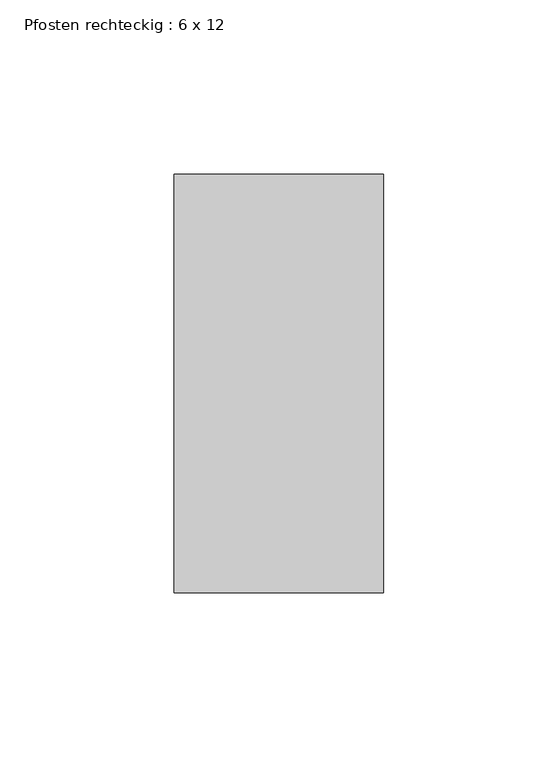
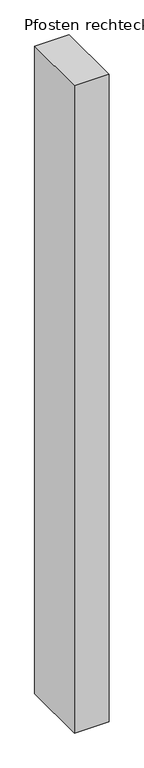
"""IFC4 building model written with IfcOpenShell, lengths in millimetres: member geometry, Pfosten rechteckig : 6 x 12."""

import ifcopenshell
import ifcopenshell.guid

model = None  # the IFC model being written
_history = None  # IfcOwnerHistory: only IFC2X3 demands one
_inside = {}  # id of a spatial element -> (the spatial element, [elements in it])
_under = {}  # id of a project, library or spatial element -> (it, [spatial elements below it])
_declared = {}  # id of a project -> (the project, [libraries it declares])
_typed = {}  # id of a type object -> (the type object, [elements of that type])
_made_of = {}  # id of a material, layer set ... -> (it, [elements and type objects made of it])


def new_model(schema):
    """Start an empty IFC model of exactly this schema.

    Asked for "IFC4X3", IfcOpenShell would pick the latest addendum, in which some entities
    have other attributes; the version numbers below select the first issue.
    IFC2X3 requires an IfcOwnerHistory on every rooted entity: one is made here for all.
    """
    global model, _history
    if schema == "IFC4X3":
        model = ifcopenshell.file(schema_version=(4, 3, 0, 0))
    else:
        model = ifcopenshell.file(schema=schema)
    _inside.clear()
    _under.clear()
    _declared.clear()
    _typed.clear()
    _made_of.clear()
    _history = None
    if model.schema == "IFC2X3":
        org = make("IfcOrganization", Name="unknown")
        user = make(
            "IfcPersonAndOrganization",
            ThePerson=make("IfcPerson", FamilyName="unknown"),
            TheOrganization=org,
        )
        app = make(
            "IfcApplication",
            ApplicationDeveloper=org,
            Version="unknown",
            ApplicationFullName="unknown",
            ApplicationIdentifier="unknown",
        )
        _history = make(
            "IfcOwnerHistory",
            OwningUser=user,
            OwningApplication=app,
            ChangeAction="ADDED",
            CreationDate=0,
        )
    return model


def make(cls, **values):
    """One entity of the class cls with the attributes given. An attribute that is None is left unset."""
    return model.create_entity(
        cls, **{name: value for name, value in values.items() if value is not None}
    )


def rooted(cls, **values):
    """An entity with a GlobalId (a new one), such as an element, a storey or a relation."""
    return make(cls, GlobalId=ifcopenshell.guid.new(), OwnerHistory=_history, **values)


def si_unit(unit_type, name, prefix=None):
    """IfcSIUnit, for example si_unit("LENGTHUNIT", "METRE", prefix="MILLI")."""
    return make("IfcSIUnit", UnitType=unit_type, Prefix=prefix, Name=name)


def assignment(units):
    """IfcUnitAssignment: the units of a project."""
    return None if units is None else make("IfcUnitAssignment", Units=units)


def point(xyz):
    """IfcCartesianPoint."""
    return None if xyz is None else make("IfcCartesianPoint", Coordinates=xyz)


def direction(xyz):
    """IfcDirection."""
    return None if xyz is None else make("IfcDirection", DirectionRatios=xyz)


def frame(location, z_axis=None, x_axis=None):
    """IfcAxis2Placement3D, a coordinate frame: its origin and axes. An axis left out is left unset."""
    return make(
        "IfcAxis2Placement3D",
        Location=point(location),
        Axis=direction(z_axis),
        RefDirection=direction(x_axis),
    )


def origin():
    """The frame at (0, 0, 0) with its axes left unset."""
    return frame((0.0, 0.0, 0.0))


def place(relative_to, where):
    """IfcLocalPlacement: puts the frame where relative to a parent placement (None: the world)."""
    return make(
        "IfcLocalPlacement", PlacementRelTo=relative_to, RelativePlacement=where
    )


def context(
    kind, dimensions, precision=None, world=None, true_north=None, identifier=None
):
    """IfcGeometricRepresentationContext, for example the 3D "Model" context."""
    return make(
        "IfcGeometricRepresentationContext",
        ContextIdentifier=identifier,
        ContextType=kind,
        CoordinateSpaceDimension=dimensions,
        Precision=precision,
        WorldCoordinateSystem=world,
        TrueNorth=true_north,
    )


def project(units=None, contexts=None):
    """IfcProject with its units and contexts."""
    return rooted(
        "IfcProject",
        Name="project",
        RepresentationContexts=contexts,
        UnitsInContext=assignment(units),
    )


def spatial(cls, under=None, at=None, **own):
    """A site, building, storey or space (cls), placed at a placement, below another one or the project."""
    s = rooted(cls, ObjectPlacement=at, **own)
    if under is not None:
        _under.setdefault(under.id(), (under, []))[1].append(s)
    return s


def polyline(points):
    """IfcPolyline through the points."""
    return make("IfcPolyline", Points=[point(p) for p in points])


def outline(outer, holes=None, kind="AREA"):
    """IfcArbitraryClosedProfileDef: a profile drawn as a closed curve; with holes, ...WithVoids."""
    if holes is None:
        return make("IfcArbitraryClosedProfileDef", ProfileType=kind, OuterCurve=outer)
    return make(
        "IfcArbitraryProfileDefWithVoids",
        ProfileType=kind,
        OuterCurve=outer,
        InnerCurves=holes,
    )


def extrude(swept, where, along, depth):
    """IfcExtrudedAreaSolid: the profile swept, set in the frame where, extruded along a direction by depth."""
    return make(
        "IfcExtrudedAreaSolid",
        SweptArea=swept,
        Position=where,
        ExtrudedDirection=direction(along),
        Depth=depth,
    )


def shape(context_of_items, identifier, shape_type, items):
    """IfcShapeRepresentation: the items that make up one representation, for example the "Body"."""
    return make(
        "IfcShapeRepresentation",
        ContextOfItems=context_of_items,
        RepresentationIdentifier=identifier,
        RepresentationType=shape_type,
        Items=items,
    )


def source(mapping_origin, context_of_items, identifier, shape_type, items):
    """IfcRepresentationMap: a shape defined once, which mapped items show again and again."""
    return make(
        "IfcRepresentationMap",
        MappingOrigin=mapping_origin,
        MappedRepresentation=shape(context_of_items, identifier, shape_type, items),
    )


def transform(
    local_origin,
    x_axis=None,
    y_axis=None,
    z_axis=None,
    scale=None,
    scale2=None,
    scale3=None,
    uniform=True,
):
    """IfcCartesianTransformationOperator3D, or its non-uniform kind. x_axis, y_axis, z_axis: its Axis1, 2, 3."""
    if uniform:
        return make(
            "IfcCartesianTransformationOperator3D",
            Axis1=direction(x_axis),
            Axis2=direction(y_axis),
            LocalOrigin=point(local_origin),
            Scale=scale,
            Axis3=direction(z_axis),
        )
    return make(
        "IfcCartesianTransformationOperator3DnonUniform",
        Axis1=direction(x_axis),
        Axis2=direction(y_axis),
        LocalOrigin=point(local_origin),
        Scale=scale,
        Axis3=direction(z_axis),
        Scale2=scale2,
        Scale3=scale3,
    )


def mapped(mapping_source, mapping_target):
    """IfcMappedItem: shows the shape of a source again, moved by a transform."""
    return make(
        "IfcMappedItem", MappingSource=mapping_source, MappingTarget=mapping_target
    )


def made_of(thing, what):
    """Note that an element or type object is made of a material, layer set ...; save() writes the relation."""
    if what is not None:
        _made_of.setdefault(what.id(), (what, []))[1].append(thing)
    return thing


def element(
    cls,
    number,
    at=None,
    inside=None,
    cuts=None,
    type_object=None,
    material=None,
    context=None,
    identifier="Body",
    shape_type=None,
    held_by="IfcProductDefinitionShape",
    body=None,
    shapes=None,
    **own,
):
    """One element of the class cls, such as IfcWall. Its Tag is "e" and its number.

    at: its placement. inside: the storey or other place that contains it. cuts: it is an
    opening in that element (IfcRelVoidsElement). A single representation is given by context,
    identifier, shape_type and body (its items); several are given by shapes. held_by: the class
    of the entity that holds the representations. save() writes the other relations.
    """
    e = rooted(cls, Tag="e%d" % number, ObjectPlacement=at, **own)
    if body is not None:
        shapes = [shape(context, identifier, shape_type, body)]
    if shapes is not None:
        e.Representation = make(held_by, Representations=shapes)
    if inside is not None:
        _inside.setdefault(inside.id(), (inside, []))[1].append(e)
    if cuts is not None:
        rooted(
            "IfcRelVoidsElement", RelatingBuildingElement=cuts, RelatedOpeningElement=e
        )
    if type_object is not None:
        _typed.setdefault(type_object.id(), (type_object, []))[1].append(e)
    return made_of(e, material)


def aggregate(whole, parts):
    """IfcRelAggregates: a whole, such as a stair, and the parts it consists of."""
    return rooted("IfcRelAggregates", RelatingObject=whole, RelatedObjects=parts)


def save(model, path):
    """Write the relations noted so far, then the file.

    IfcRelAggregates (storeys below a building ...), IfcRelContainedInSpatialStructure (elements
    in a storey), IfcRelDefinesByType, IfcRelAssociatesMaterial and IfcRelDeclares: one each for
    every whole, place, type object, material and project.
    """
    for whole, parts in _under.values():
        aggregate(whole, parts)
    for where, things in _inside.values():
        rooted(
            "IfcRelContainedInSpatialStructure",
            RelatedElements=things,
            RelatingStructure=where,
        )
    for kind, things in _typed.values():
        rooted("IfcRelDefinesByType", RelatedObjects=things, RelatingType=kind)
    for what, things in _made_of.values():
        rooted("IfcRelAssociatesMaterial", RelatedObjects=things, RelatingMaterial=what)
    for by, libraries in _declared.values():
        rooted("IfcRelDeclares", RelatingContext=by, RelatedDefinitions=libraries)
    model.write(path)


def pfosten_rechteckig_6_x_12_8bb825ca(model_context):
    return source(origin(), model_context, "Body", "SweptSolid", [
        extrude(outline(polyline([(30.0, 60.0), (30.0, -60.0), (-30.0, -60.0), (-30.0, 60.0), (30.0, 60.0)])), frame((0.0, 0.0, -1190.0), z_axis=(0.0, 0.0, 1.0), x_axis=(1.0, 0.0, 0.0)), (0.0, 0.0, 1.0), 1190.0),
    ])


if __name__ == "__main__":
    model = new_model("IFC4")
    model_context = context("Model", 3, world=origin())
    ifc_project = project(units=[si_unit("LENGTHUNIT", "METRE", prefix="MILLI")], contexts=[model_context])
    site = spatial("IfcSite", under=ifc_project)
    building = spatial("IfcBuilding", under=site)
    placement = place(None, origin())
    pfosten_rechteckig_6_x_12_shape = pfosten_rechteckig_6_x_12_8bb825ca(model_context)
    element("IfcMember", 1, ObjectType="Pfosten rechteckig : 6 x 12", at=placement, inside=building, context=model_context, shape_type="MappedRepresentation", body=[
        mapped(pfosten_rechteckig_6_x_12_shape, transform((0.0, 0.0, 0.0), x_axis=(1.0, 0.0, 0.0), y_axis=(0.0, 1.0, 0.0), z_axis=(0.0, 0.0, 1.0))),
    ])
    save(model, "model.ifc")

# Revit data of these elements
# Type "Pfosten rechteckig : 6 x 12"
#   built-in parameter 1007304 = 0.393701 (stored number, unit not read)
#   built-in parameter 1007301 = 0.0984252 (stored number, unit not read)
#   built-in parameter 1007300 = 0.0984252 (stored number, unit not read)
# Element 1 (IfcMember, "Pfosten rechteckig : 6 x 12")
#   Materials on its faces: "Metall - verzinkt"
# Materials
#   "Metall - verzinkt": class "Allgemeines", colour RGB 200 200 200, transparency 0, Cost = 0
